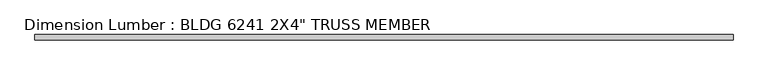
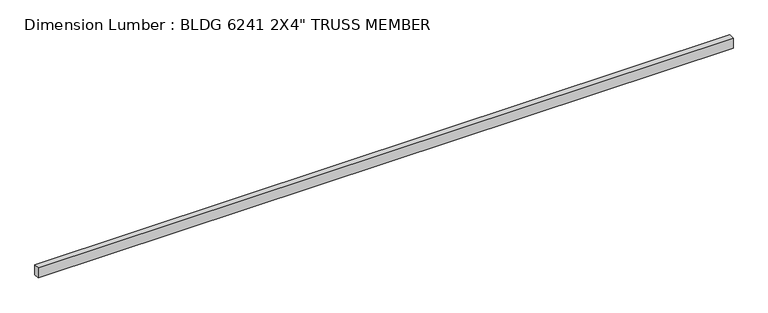
"""IFC4 building model written with IfcOpenShell, lengths in millimetres: beam geometry."""

from ifc_helpers import new_model, si_unit, frame, origin, place, context, project, spatial, polyline, outline, extrude, source, transform, mapped, element, save


def beam_4ff5e491(model_context):
    return source(origin(), model_context, "Body", "SweptSolid", [
        extrude(outline(polyline([(3248.0249994, 25.4), (3248.0249994, -25.4), (-3248.0249994, -25.4), (-3248.0249994, 25.4), (3248.0249994, 25.4)])), frame((0.0, 0.0, -50.8), z_axis=(0.0, 0.0, 1.0), x_axis=(1.0, 0.0, 0.0)), (0.0, 0.0, 1.0), 101.6),
    ])


if __name__ == "__main__":
    model = new_model("IFC4")
    model_context = context("Model", 3, world=origin())
    ifc_project = project(units=[si_unit("LENGTHUNIT", "METRE", prefix="MILLI")], contexts=[model_context])
    site = spatial("IfcSite", under=ifc_project)
    building = spatial("IfcBuilding", under=site)
    placement = place(None, origin())
    beam_shape = beam_4ff5e491(model_context)
    element("IfcBeam", 1, ObjectType="Dimension Lumber : BLDG 6241 2X4\" TRUSS MEMBER", at=placement, inside=building, context=model_context, shape_type="MappedRepresentation", body=[
        mapped(beam_shape, transform((0.0, 0.0, 0.0), x_axis=(1.0, 0.0, 0.0), y_axis=(0.0, 1.0, 0.0), z_axis=(0.0, 0.0, 1.0))),
    ])
    save(model, "model.ifc")

# Revit data of these elements
# Type "Dimension Lumber : BLDG 6241 2X4\" TRUSS MEMBER"
#   Assembly Code = "B10"
#   A = 0.273472 SF
#   Length [instance default] = 5' - 0"
#   b = 0' - 2"
#   d = 0' - 4"
#   Structural Material [instance default] = Softwood, Lumber
# Element 1 (IfcBeam, "Dimension Lumber : BLDG 6241 2X4\" TRUSS MEMBER")
#   Materials on its faces: "Softwood, Lumber"
# Materials
#   "Softwood, Lumber": class "Wood", colour RGB 223 192 134, transparency 0, Description = "Pinus Echinata", Cost = 0
